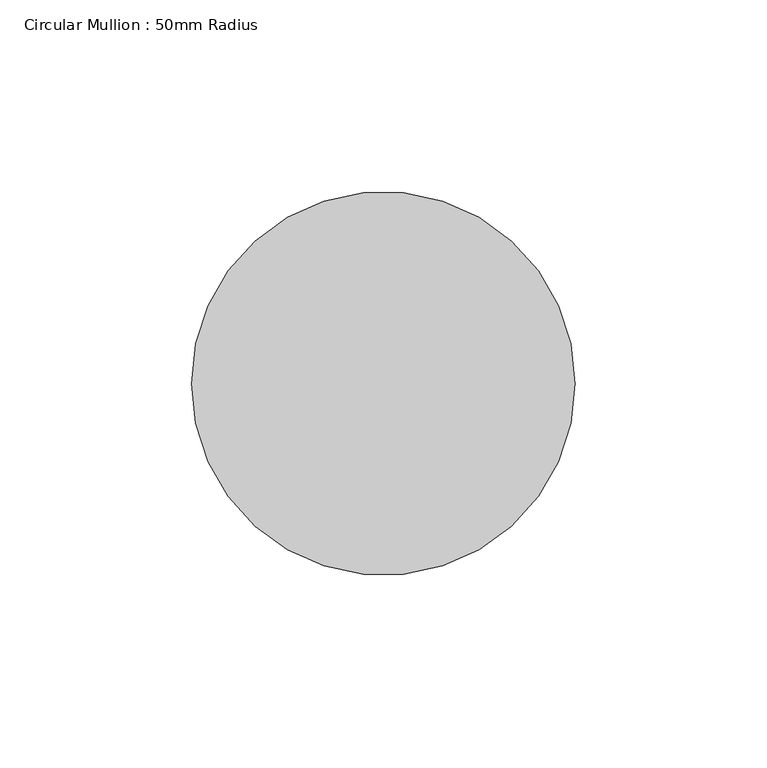
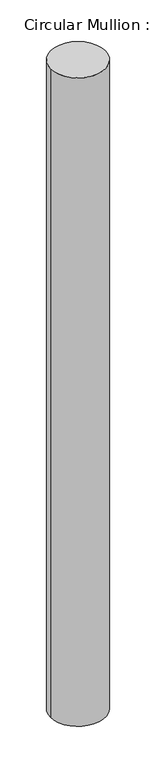
"""IFC4 building model written with IfcOpenShell, lengths in millimetres: member geometry, Circular Mullion : 50mm Radius."""

from ifc_helpers import new_model, si_unit, point, frame, origin, origin_2d, place, context, project, spatial, circle_curve, trimmed, segment, composite_curve, outline, extrude, source, transform, mapped, element, save


def circular_mullion_50mm_radius_5df7566e(model_context):
    return source(origin(), model_context, "Body", "SweptSolid", [
        extrude(outline(composite_curve([segment(trimmed(circle_curve(origin_2d(), 50.0), [point((50.0, 0.0))], [point((-50.0, 0.0))], False, "CARTESIAN"), True, "CONTINUOUS"), segment(trimmed(circle_curve(origin_2d(), 50.0), [point((-50.0, 0.0))], [point((50.0, 0.0))], False, "CARTESIAN"), True, "CONTINUOUS")], self_intersect=False)), frame((0.0, 0.0, -1247.6926488), z_axis=(0.0, 0.0, 1.0), x_axis=(1.0, 0.0, 0.0)), (0.0, 0.0, 1.0), 1247.6926488),
    ])


if __name__ == "__main__":
    model = new_model("IFC4")
    model_context = context("Model", 3, world=origin())
    ifc_project = project(units=[si_unit("LENGTHUNIT", "METRE", prefix="MILLI")], contexts=[model_context])
    site = spatial("IfcSite", under=ifc_project)
    building = spatial("IfcBuilding", under=site)
    placement = place(None, origin())
    circular_mullion_50mm_radius_shape = circular_mullion_50mm_radius_5df7566e(model_context)
    element("IfcMember", 1, ObjectType="Circular Mullion : 50mm Radius", at=placement, inside=building, context=model_context, shape_type="MappedRepresentation", body=[
        mapped(circular_mullion_50mm_radius_shape, transform((0.0, 0.0, 0.0), x_axis=(1.0, 0.0, 0.0), y_axis=(0.0, 1.0, 0.0), z_axis=(0.0, 0.0, 1.0))),
    ])
    save(model, "model.ifc")

# Revit data of these elements
# Type "Circular Mullion : 50mm Radius"
#   built-in parameter 1007350 = 0.164042 (stored number, unit not read)
# Element 1 (IfcMember, "Circular Mullion : 50mm Radius")
#   Materials on its faces: "Aluminium"
# Materials
#   "Aluminium": class "Metal", colour RGB 247 247 247, transparency 0, Description = "Aluminium 6061", Cost = 0
